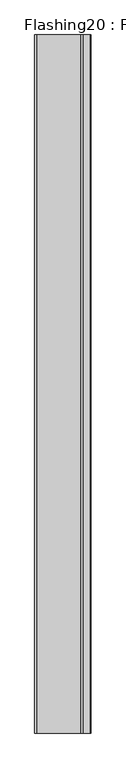
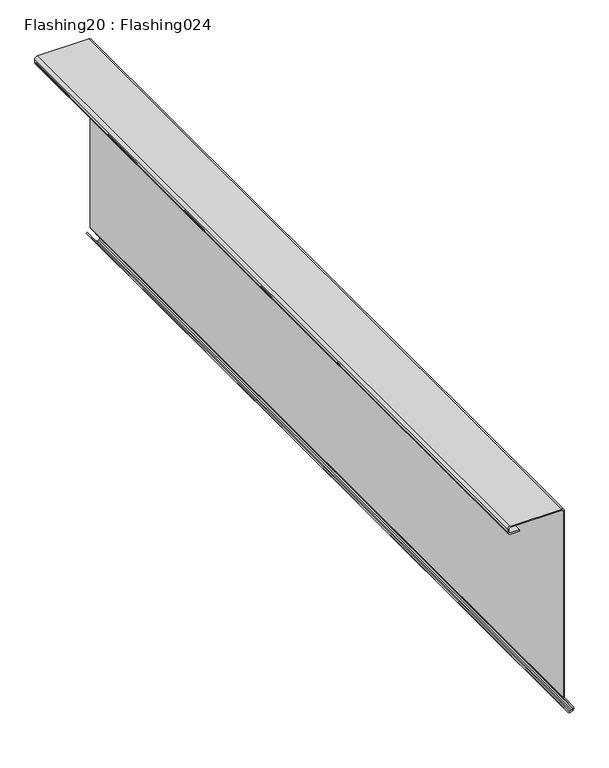
"""IFC4 building model written with IfcOpenShell, lengths in millimetres: proxy geometry, Flashing20 : Flashing024."""

from ifc_helpers import new_model, si_unit, point, frame, frame_2d, origin, place, context, project, spatial, polyline, circle_curve, trimmed, segment, composite_curve, outline, extrude, source, transform, mapped, element, save


def flashing20_flashing024_9ad17ddb(model_context):
    return source(origin(), model_context, "Body", "SweptSolid", [
        extrude(outline(composite_curve([segment(trimmed(circle_curve(frame_2d((41323.8783762, 6183.9556944)), 6.35), [point((41320.2092308, 6178.7730434))], [point((41318.4012804, 6187.1687804))], False, "CARTESIAN"), True, "CONTINUOUS"), segment(polyline([(41318.4012804, 6187.1687804), (41320.1425067, 6190.1369125)]), True, "CONTINUOUS"), segment(trimmed(circle_curve(frame_2d((41325.6196026, 6186.9238265)), 6.35), [point((41320.1425067, 6190.1369125))], [point((41329.2370767, 6192.1426751))], False, "CARTESIAN"), True, "CONTINUOUS"), segment(polyline([(41329.2370767, 6192.1426751), (41359.2301171, 6171.3528311)]), True, "CONTINUOUS"), segment(trimmed(circle_curve(frame_2d((41362.8475913, 6176.5716797)), 6.35), [point((41359.2301171, 6171.3528311))], [point((41362.8475913, 6170.2216797))], True, "CARTESIAN"), True, "CONTINUOUS"), segment(polyline([(41362.8475913, 6170.2216797), (41842.9189039, 6170.2216797)]), True, "CONTINUOUS"), segment(trimmed(circle_curve(frame_2d((41842.9189039, 6163.8716797)), 6.35), [point((41842.9189039, 6170.2216797))], [point((41849.2689039, 6163.8716797))], False, "CARTESIAN"), True, "CONTINUOUS"), segment(polyline([(41849.2689039, 6163.8716797), (41849.2689039, 6038.1540605)]), True, "CONTINUOUS"), segment(trimmed(circle_curve(frame_2d((41842.9189039, 6038.1540605)), 6.35), [point((41849.2689039, 6038.1540605))], [point((41842.9189039, 6031.8040605))], False, "CARTESIAN"), True, "CONTINUOUS"), segment(polyline([(41842.9189039, 6031.8040605), (41835.0524976, 6031.8040605)]), True, "CONTINUOUS"), segment(trimmed(circle_curve(frame_2d((41835.0524976, 6038.1540605)), 6.35), [point((41835.0524976, 6031.8040605))], [point((41828.7024976, 6038.1540605))], False, "CARTESIAN"), True, "CONTINUOUS"), segment(polyline([(41828.7024976, 6038.1540605), (41828.7024976, 6060.1805253), (41831.7024976, 6060.1805253), (41831.7024976, 6038.1540605)]), True, "CONTINUOUS"), segment(trimmed(circle_curve(frame_2d((41835.0524976, 6038.1540605)), 3.35), [point((41831.7024976, 6038.1540605))], [point((41835.0524976, 6034.8040605))], True, "CARTESIAN"), True, "CONTINUOUS"), segment(polyline([(41835.0524976, 6034.8040605), (41842.9189039, 6034.8040605)]), True, "CONTINUOUS"), segment(trimmed(circle_curve(frame_2d((41842.9189039, 6038.1540605)), 3.35), [point((41842.9189039, 6034.8040605))], [point((41846.2689039, 6038.1540605))], True, "CARTESIAN"), True, "CONTINUOUS"), segment(polyline([(41846.2689039, 6038.1540605), (41846.2689039, 6163.8716797)]), True, "CONTINUOUS"), segment(trimmed(circle_curve(frame_2d((41842.9189039, 6163.8716797)), 3.35), [point((41846.2689039, 6163.8716797))], [point((41842.9189039, 6167.2216797))], True, "CARTESIAN"), True, "CONTINUOUS"), segment(polyline([(41842.9189039, 6167.2216797), (41362.8475913, 6167.2216797)]), True, "CONTINUOUS"), segment(trimmed(circle_curve(frame_2d((41362.8475913, 6176.5716797)), 9.35), [point((41362.8475913, 6167.2216797))], [point((41357.5210742, 6168.8872333))], False, "CARTESIAN"), True, "CONTINUOUS"), segment(polyline([(41357.5210742, 6168.8872333), (41327.5280338, 6189.6770774)]), True, "CONTINUOUS"), segment(trimmed(circle_curve(frame_2d((41325.6196026, 6186.9238265)), 3.35), [point((41327.5280338, 6189.6770774))], [point((41322.730111, 6188.6189191))], True, "CARTESIAN"), True, "CONTINUOUS"), segment(polyline([(41322.730111, 6188.6189191), (41320.9888847, 6185.650787)]), True, "CONTINUOUS"), segment(trimmed(circle_curve(frame_2d((41323.8783762, 6183.9556944)), 3.35), [point((41320.9888847, 6185.650787))], [point((41321.9426853, 6181.2215399))], True, "CARTESIAN"), True, "CONTINUOUS"), segment(polyline([(41321.9426853, 6181.2215399), (41352.3883692, 6159.6670035), (41350.6549147, 6157.218507), (41320.2092308, 6178.7730434)]), True, "CONTINUOUS")], self_intersect=False)), frame((0.0, 2217.3609988, 0.0), z_axis=(0.0, 1.0, 0.0), x_axis=(0.0, 0.0, 1.0)), (0.0, 0.0, 1.0), 2000.0),
    ])


if __name__ == "__main__":
    model = new_model("IFC4")
    model_context = context("Model", 3, world=origin())
    ifc_project = project(units=[si_unit("LENGTHUNIT", "METRE", prefix="MILLI")], contexts=[model_context])
    site = spatial("IfcSite", under=ifc_project)
    building = spatial("IfcBuilding", under=site)
    placement = place(None, origin())
    flashing20_flashing024_shape = flashing20_flashing024_9ad17ddb(model_context)
    element("IfcBuildingElementProxy", 1, Name="Flashing20 : Flashing024", ObjectType="Flashing20 : Flashing024", at=placement, inside=building, context=model_context, shape_type="MappedRepresentation", body=[
        mapped(flashing20_flashing024_shape, transform((0.0, 0.0, 0.0), x_axis=(1.0, 0.0, 0.0), y_axis=(0.0, 1.0, 0.0), z_axis=(0.0, 0.0, 1.0))),
    ])
    save(model, "model.ifc")

# Revit data of these elements
# Type "Flashing20 : Flashing024"
#   NameOverride = "Flashing024"
# Element 1 (IfcBuildingElementProxy, "Flashing20 : Flashing024")
#   Materials on its faces: "BRAKE METAL EAVE TRIM TO MATCH STANDING SEAM COLOR"
# Materials
#   "BRAKE METAL EAVE TRIM TO MATCH STANDING SEAM COLOR": class "Unassigned", colour RGB 128 128 128, transparency 0, Cost = 0
